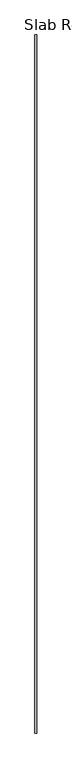
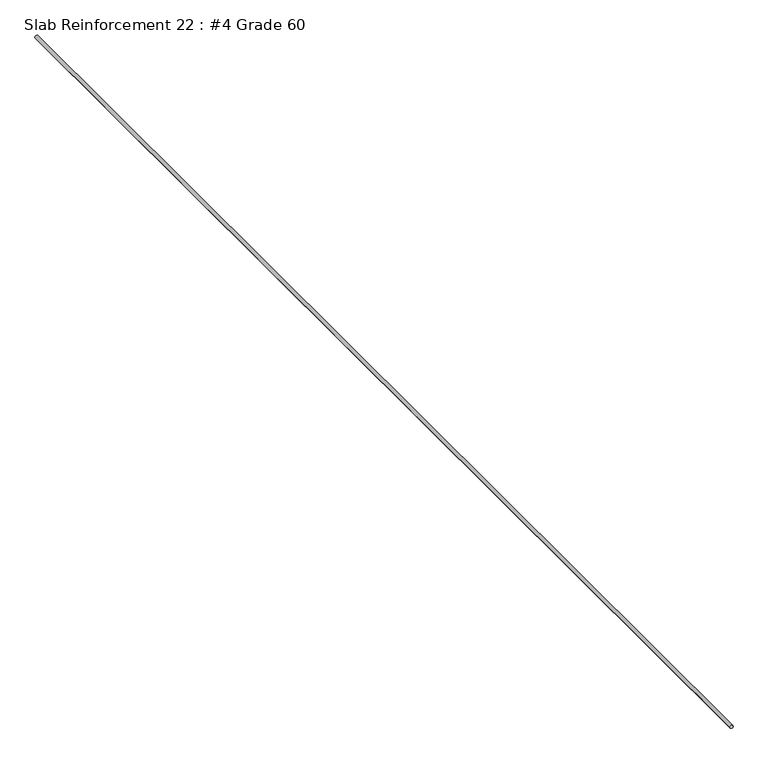
"""IFC4 building model written with IfcOpenShell, lengths in millimetres: proxy geometry, Slab Reinforcement 22 : #4 Grade 60."""

from ifc_helpers import new_model, si_unit, point, frame, frame_2d, origin, place, context, project, spatial, circle_curve, trimmed, segment, composite_curve, outline, extrude, source, transform, mapped, element, save


def slab_reinforcement_22_4_grade_60_b1e4fe1f(model_context):
    return source(origin(), model_context, "Body", "SweptSolid", [
        extrude(outline(composite_curve([segment(trimmed(circle_curve(frame_2d((-69.85, 588840.1672365)), 6.35), [point((-69.85, 588833.8172365))], [point((-69.85, 588846.5172365))], False, "CARTESIAN"), True, "CONTINUOUS"), segment(trimmed(circle_curve(frame_2d((-69.85, 588840.1672365)), 6.35), [point((-69.85, 588846.5172365))], [point((-69.85, 588833.8172365))], False, "CARTESIAN"), True, "CONTINUOUS")], self_intersect=False)), frame((0.0, -536411.2413841, 0.0), z_axis=(0.0, 1.0, 0.0), x_axis=(0.0, 0.0, 1.0)), (0.0, 0.0, 1.0), 4724.4),
    ])


if __name__ == "__main__":
    model = new_model("IFC4")
    model_context = context("Model", 3, world=origin())
    ifc_project = project(units=[si_unit("LENGTHUNIT", "METRE", prefix="MILLI")], contexts=[model_context])
    site = spatial("IfcSite", under=ifc_project)
    building = spatial("IfcBuilding", under=site)
    placement = place(None, origin())
    slab_reinforcement_22_4_grade_60_shape = slab_reinforcement_22_4_grade_60_b1e4fe1f(model_context)
    element("IfcBuildingElementProxy", 1, Name="Slab Reinforcement 22 : #4 Grade 60", ObjectType="Slab Reinforcement 22 : #4 Grade 60", at=placement, inside=building, context=model_context, shape_type="MappedRepresentation", body=[
        mapped(slab_reinforcement_22_4_grade_60_shape, transform((0.0, 0.0, 0.0), x_axis=(1.0, 0.0, 0.0), y_axis=(0.0, 1.0, 0.0), z_axis=(0.0, 0.0, 1.0))),
    ])
    save(model, "model.ifc")

# Revit data of these elements
# Element 1 (IfcBuildingElementProxy, "Slab Reinforcement 22 : #4 Grade 60")
#   Materials on its faces: "#4 GR. 60 REINF. @ 16\" O.C. EW."
# Materials
#   "#4 GR. 60 REINF. @ 16\" O.C. EW.": class "Generic", colour RGB 84 83 81, transparency 0, Cost = 0
